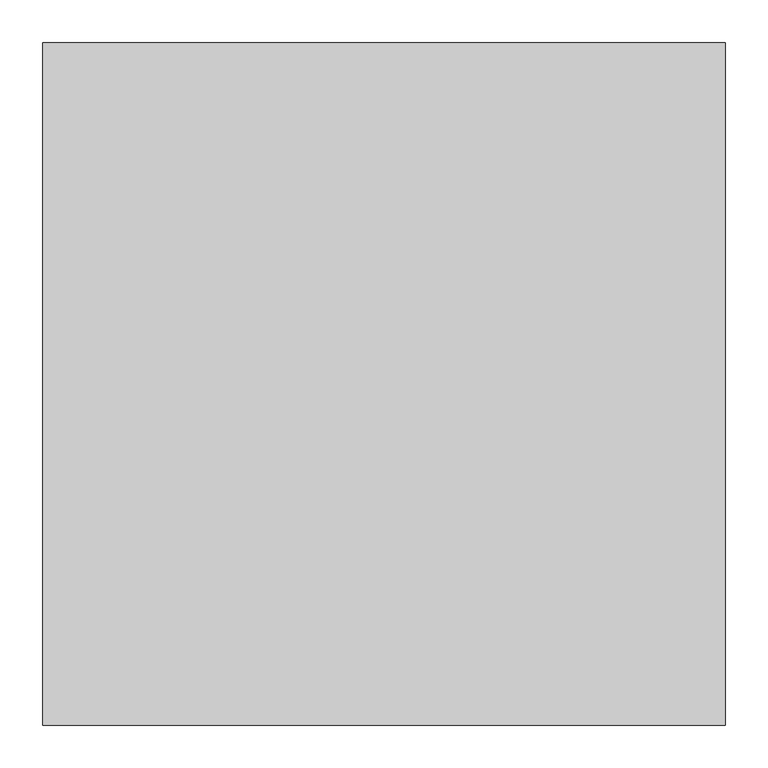
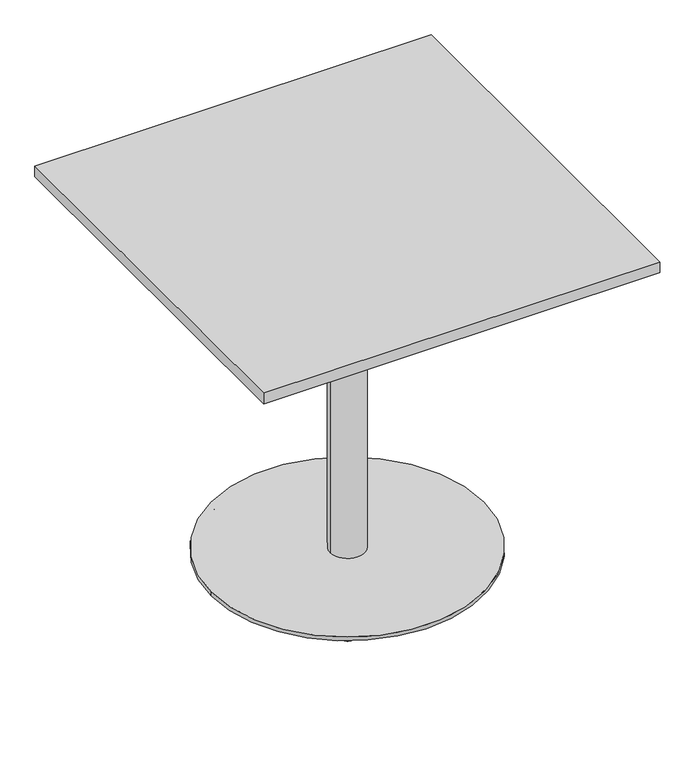
"""IFC4 building model written with IfcOpenShell, lengths in millimetres: furniture geometry, U-MCZZR81N : U-MCZZR81N."""

from ifc_helpers import new_model, si_unit, point, frame, frame_2d, origin, origin_with_axes, origin_2d, place, context, project, spatial, polyline, circle_curve, trimmed, segment, composite_curve, outline, extrude, source, transform, mapped, element, save


def furniture_5036bc18(model_context):
    return source(origin(), model_context, "Body", "SweptSolid", [
        extrude(outline(composite_curve([segment(trimmed(circle_curve(frame_2d((-255.0001777, 0.0)), 12.5), [point((-267.5001777, 0.0))], [point((-242.5001777, 0.0))], False, "CARTESIAN"), True, "CONTINUOUS"), segment(trimmed(circle_curve(frame_2d((-255.0001777, 0.0)), 12.5), [point((-242.5001777, 0.0))], [point((-267.5001777, 0.0))], False, "CARTESIAN"), True, "CONTINUOUS")], self_intersect=False)), origin_with_axes(), (0.0, 0.0, 1.0), 6.0),
        extrude(outline(composite_curve([segment(trimmed(circle_curve(frame_2d((-127.5000664, 220.835939)), 12.5), [point((-140.0000664, 220.835939))], [point((-115.0000664, 220.835939))], False, "CARTESIAN"), True, "CONTINUOUS"), segment(trimmed(circle_curve(frame_2d((-127.5000664, 220.835939)), 12.5), [point((-115.0000664, 220.835939))], [point((-140.0000664, 220.835939))], False, "CARTESIAN"), True, "CONTINUOUS")], self_intersect=False)), origin_with_axes(), (0.0, 0.0, 1.0), 6.0),
        extrude(outline(composite_curve([segment(trimmed(circle_curve(frame_2d((127.5000664, 220.835939)), 12.5), [point((115.0000664, 220.835939))], [point((140.0000664, 220.835939))], False, "CARTESIAN"), True, "CONTINUOUS"), segment(trimmed(circle_curve(frame_2d((127.5000664, 220.835939)), 12.5), [point((140.0000664, 220.835939))], [point((115.0000664, 220.835939))], False, "CARTESIAN"), True, "CONTINUOUS")], self_intersect=False)), origin_with_axes(), (0.0, 0.0, 1.0), 6.0),
        extrude(outline(composite_curve([segment(trimmed(circle_curve(frame_2d((255.0001777, 0.0)), 12.5), [point((242.5001777, 0.0))], [point((267.5001777, 0.0))], False, "CARTESIAN"), True, "CONTINUOUS"), segment(trimmed(circle_curve(frame_2d((255.0001777, 0.0)), 12.5), [point((267.5001777, 0.0))], [point((242.5001777, 0.0))], False, "CARTESIAN"), True, "CONTINUOUS")], self_intersect=False)), origin_with_axes(), (0.0, 0.0, 1.0), 6.0),
        extrude(outline(composite_curve([segment(trimmed(circle_curve(frame_2d((-127.5000664, -220.835939)), 12.5), [point((-140.0000664, -220.835939))], [point((-115.0000664, -220.835939))], False, "CARTESIAN"), True, "CONTINUOUS"), segment(trimmed(circle_curve(frame_2d((-127.5000664, -220.835939)), 12.5), [point((-115.0000664, -220.835939))], [point((-140.0000664, -220.835939))], False, "CARTESIAN"), True, "CONTINUOUS")], self_intersect=False)), origin_with_axes(), (0.0, 0.0, 1.0), 6.0),
        extrude(outline(composite_curve([segment(trimmed(circle_curve(frame_2d((127.5000664, -220.835939)), 12.5), [point((115.0000664, -220.835939))], [point((140.0000664, -220.835939))], False, "CARTESIAN"), True, "CONTINUOUS"), segment(trimmed(circle_curve(frame_2d((127.5000664, -220.835939)), 12.5), [point((140.0000664, -220.835939))], [point((115.0000664, -220.835939))], False, "CARTESIAN"), True, "CONTINUOUS")], self_intersect=False)), origin_with_axes(), (0.0, 0.0, 1.0), 6.0),
        extrude(outline(composite_curve([segment(trimmed(circle_curve(origin_2d(), 35.0), [point((35.0, 0.0))], [point((-35.0, 0.0))], False, "CARTESIAN"), True, "CONTINUOUS"), segment(trimmed(circle_curve(origin_2d(), 35.0), [point((-35.0, 0.0))], [point((35.0, 0.0))], False, "CARTESIAN"), True, "CONTINUOUS")], self_intersect=False)), frame((0.0, 0.0, 14.0), z_axis=(0.0, 0.0, 1.0), x_axis=(1.0, 0.0, 0.0)), (0.0, 0.0, 1.0), 688.0),
        extrude(outline(composite_curve([segment(trimmed(circle_curve(origin_2d(), 275.0), [point((275.0, 0.0))], [point((-275.0, 0.0))], False, "CARTESIAN"), True, "CONTINUOUS"), segment(trimmed(circle_curve(origin_2d(), 275.0), [point((-275.0, 0.0))], [point((275.0, 0.0))], False, "CARTESIAN"), True, "CONTINUOUS")], self_intersect=False)), frame((0.0, 0.0, 6.0), z_axis=(0.0, 0.0, 1.0), x_axis=(1.0, 0.0, 0.0)), (0.0, 0.0, 1.0), 8.0),
        extrude(outline(polyline([(400.0, 400.0), (400.0, -400.0), (-400.0, -400.0), (-400.0, 400.0), (400.0, 400.0)])), frame((0.0, 0.0, 702.0), z_axis=(0.0, 0.0, 1.0), x_axis=(1.0, 0.0, 0.0)), (0.0, 0.0, 1.0), 23.0),
    ])


if __name__ == "__main__":
    model = new_model("IFC4")
    model_context = context("Model", 3, world=origin())
    ifc_project = project(units=[si_unit("LENGTHUNIT", "METRE", prefix="MILLI")], contexts=[model_context])
    site = spatial("IfcSite", under=ifc_project)
    building = spatial("IfcBuilding", under=site)
    placement = place(None, origin())
    furniture_shape = furniture_5036bc18(model_context)
    element("IfcFurniture", 1, ObjectType="U-MCZZR81N : U-MCZZR81N", at=placement, inside=building, context=model_context, shape_type="MappedRepresentation", body=[
        mapped(furniture_shape, transform((0.0, 0.0, 0.0), x_axis=(1.0, 0.0, 0.0), y_axis=(0.0, 1.0, 0.0), z_axis=(0.0, 0.0, 1.0))),
    ])
    save(model, "model.ifc")

# Revit data of these elements
# Type "U-MCZZR81N : U-MCZZR81N"
#   Youtube clip = ""
#   Weight Net (kg) = ""
#   WarrantyStartDate = ""
#   WarrantyDuration = ""
#   Uniclass 2.0 Description = "Desks, Tables And Worktops"
#   Uniclass 2.0 Code = "PR-31-22"
#   Uniclass 1.4 Description = "Conference room furniture"
#   Uniclass 1.4 Code = "L8536"
#   URL = "http://kinnarps.bimobject.com/U-MCZZR81N"
#   UNSPSC Category = "Furniture and Furnishings"
#   TypeName = "U-MCZZR81N"
#   Technical description = "http://www.kinnarps.com/en/International/ProductsInspiration/Office/ConferenceTables/Product/?prodid=305786"
#   TagNumber = ""
#   Size = ""
#   SerialNumber = ""
#   Product identifier = "kinnarps.bimobject.com/U-MCZZR81N"
#   Product group = "MULTICOM"
#   Product family = "Conference tables"
#   Product data url = "http://www.kinnarps.com/en/International/ProductsInspiration/Office/ConferenceTables/Product/?prodid=305786"
#   Product SKU = "U-MCZZR81N"
#   Omniclass = "23.40.70.14.64.11"
#   NominalWidth = ""
#   NominalHeight = ""
#   Name of the object = "MULTICOM U-MCZZR81N"
#   NBS Reference Description = "Desks, Tables And Worktops"
#   NBS Reference = "31-22"
#   Model = "MULTICOM U-MCZZR81N"
#   Material = ""
#   Manufacturer country = "Sweden"
#   Manufacturer URL = "http://www.kinnarps.com"
#   Manufacturer = "Kinnarps"
#   InstallationDate = ""
#   Installation instructions = "http://www.kinnarps.com/en/International/ProductsInspiration/Office/ConferenceTables/Product/?prodid=305786"
#   IFC Classification = "Furniture"
#   Grade = ""
#   Finish = ""
#   Features = ""
#   Extidentifier = ""
#   Edition number = "1"
#   EAN code = ""
#   Design country = "Sweden"
#   Date of publishing = ""
#   Created on = ""
#   Created by = ""
#   ConnectionType = ""
#   Colour = ""
#   COBIe Type Category = ""
#   Barcode = ""
#   BIMobject QR code url = "http://kinnarps.bimobject.com/U-MCZZR81N"
#   BIMobject Category = "Office Furniture"
#   AssetIdentifier = ""
#   AccessibilityPerformance = ""
#   Width (mm) = 800 mm
#   Offset = 0 mm
#   Height (mm) = 725 mm
#   Depth (mm) = 800 mm
#   UNSPSC Code = 56
#   Table Top [instance default] = Kinnarps-Laminate-Beech
#   Table Leg [instance default] = Kinnarps-Metal-White
#   Material secondary = Steel
#   Material main = Wood
#   Default Elevation = 0
# Element 1 (IfcFurniture, "U-MCZZR81N : U-MCZZR81N")
#   Table Top = Kinnarps-Laminate-White
#   Materials on its faces: "Kinnarps-Plastic-Black", "Kinnarps-Metal-White", "Kinnarps-Laminate-White"
# Materials
#   "Kinnarps-Laminate-Beech": class "Miscellaneous", colour RGB 174 140 106, transparency 0
#   "Kinnarps-Metal-White": class "Miscellaneous", colour RGB 255 255 255, transparency 0
#   "Steel": class "Metal", colour RGB 189 187 185, transparency 0, Cost = 0
#   "Wood": class "Miscellaneous", colour RGB 127 127 127, transparency 0
#   "Kinnarps-Plastic-Black": class "Miscellaneous", colour RGB 0 0 0, transparency 0
#   "Kinnarps-Laminate-White": class "Miscellaneous", colour RGB 255 255 255, transparency 0
